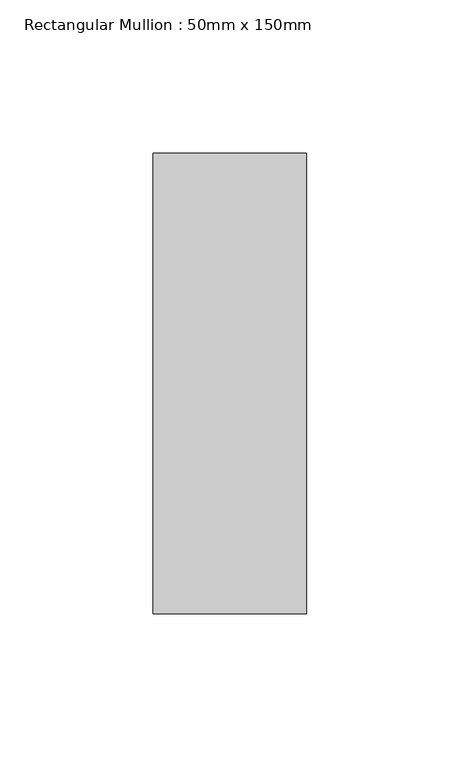
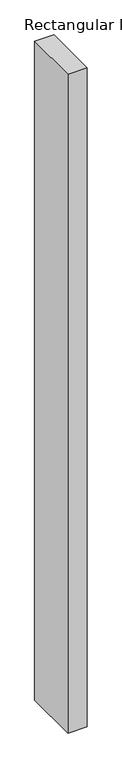
"""IFC4 building model written with IfcOpenShell, lengths in millimetres: member geometry, Rectangular Mullion : 50mm x 150mm."""

from ifc_helpers import new_model, si_unit, frame, origin, place, context, project, spatial, polyline, outline, extrude, source, transform, mapped, element, save


def rectangular_mullion_50mm_x_150mm_48da5a04(model_context):
    return source(origin(), model_context, "Body", "SweptSolid", [
        extrude(outline(polyline([(25.0, 75.0), (25.0, -75.0), (-25.0, -75.0), (-25.0, 75.0), (25.0, 75.0)])), frame((0.0, 0.0, -1822.3836314), z_axis=(0.0, 0.0, 1.0), x_axis=(1.0, 0.0, 0.0)), (0.0, 0.0, 1.0), 1822.3836314),
    ])


if __name__ == "__main__":
    model = new_model("IFC4")
    model_context = context("Model", 3, world=origin())
    ifc_project = project(units=[si_unit("LENGTHUNIT", "METRE", prefix="MILLI")], contexts=[model_context])
    site = spatial("IfcSite", under=ifc_project)
    building = spatial("IfcBuilding", under=site)
    placement = place(None, origin())
    rectangular_mullion_50mm_x_150mm_shape = rectangular_mullion_50mm_x_150mm_48da5a04(model_context)
    element("IfcMember", 1, ObjectType="Rectangular Mullion : 50mm x 150mm", at=placement, inside=building, context=model_context, shape_type="MappedRepresentation", body=[
        mapped(rectangular_mullion_50mm_x_150mm_shape, transform((0.0, 0.0, 0.0), x_axis=(1.0, 0.0, 0.0), y_axis=(0.0, 1.0, 0.0), z_axis=(0.0, 0.0, 1.0))),
    ])
    save(model, "model.ifc")

# Revit data of these elements
# Type "Rectangular Mullion : 50mm x 150mm"
#   built-in parameter 1007304 = 0.492126 (stored number, unit not read)
#   built-in parameter 1007301 = 0.082021 (stored number, unit not read)
#   built-in parameter 1007300 = 0.082021 (stored number, unit not read)
# Element 1 (IfcMember, "Rectangular Mullion : 50mm x 150mm")
#   Materials on its faces: "Aluminum"
# Materials
#   "Aluminum": class "Metal", colour RGB 244 244 244, transparency 0, Description = "Aluminum 6061", Cost = 0
